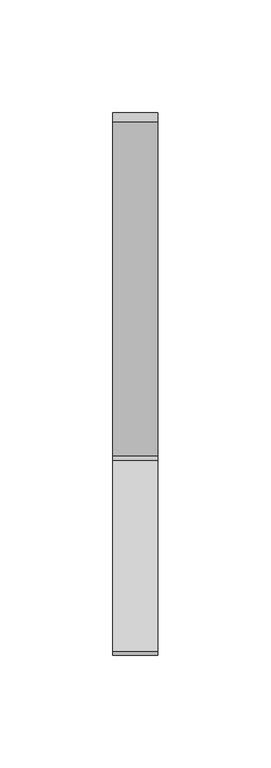
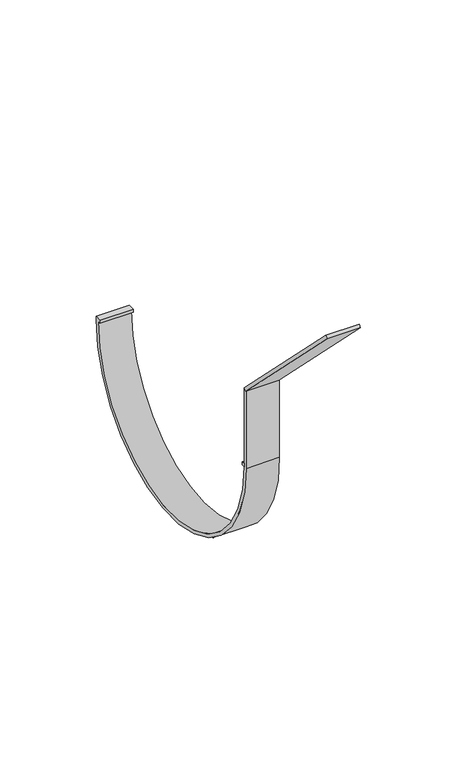
"""IFC4 building model written with IfcOpenShell, lengths in millimetres: proxy geometry, ➾ Кронштейн металлический : ➾ Кронштейн металлический."""

from ifc_helpers import new_model, si_unit, point, frame, origin, origin_with_axes, origin_2d, place, context, project, spatial, polyline, circle_curve, trimmed, segment, composite_curve, outline, extrude, source, transform, mapped, element, save


def generic_models_13adb273(model_context):
    return source(origin(), model_context, "Body", "SweptSolid", [
        extrude(outline(polyline([(0.0, -120.0), (0.0, 0.0), (20.0, 0.0), (20.0, -120.0), (0.0, -120.0)])), frame((10.0, -162.3670273, 133.4386002), z_axis=(0.0, 0.7071067811865492, 0.7071067811865459), x_axis=(-1.0, 0.0, 0.0)), (0.0, 0.0, 1.0), 2.0),
        extrude(outline(polyline([(-10.0, -74.1), (10.0, -74.1), (10.0, -76.1), (-10.0, -76.1), (-10.0, -74.1)])), origin_with_axes(), (0.0, 0.0, 1.0), 2.0),
        extrude(outline(composite_curve([segment(trimmed(circle_curve(origin_2d(), 76.1), [point((-76.1, 0.0))], [point((76.1, 0.0))], True, "CARTESIAN"), True, "CONTINUOUS"), segment(polyline([(76.1, 0.0), (74.055208, 0.0), (74.055208, 2.0), (78.1, 2.0), (78.1, 0.0)]), True, "CONTINUOUS"), segment(trimmed(circle_curve(origin_2d(), 78.1), [point((78.1, 0.0))], [point((-78.1, 0.0))], False, "CARTESIAN"), True, "CONTINUOUS"), segment(polyline([(-78.1, 0.0), (-78.1, 50.0), (-76.1, 50.0), (-76.1, 0.0)]), True, "CONTINUOUS")], self_intersect=False)), frame((-10.0, 0.0, 0.0), z_axis=(1.0, 0.0, 0.0), x_axis=(0.0, 1.0, 0.0)), (0.0, 0.0, 1.0), 20.0),
    ])


if __name__ == "__main__":
    model = new_model("IFC4")
    model_context = context("Model", 3, world=origin())
    ifc_project = project(units=[si_unit("LENGTHUNIT", "METRE", prefix="MILLI")], contexts=[model_context])
    site = spatial("IfcSite", under=ifc_project)
    building = spatial("IfcBuilding", under=site)
    placement = place(None, origin())
    generic_models_shape = generic_models_13adb273(model_context)
    element("IfcBuildingElementProxy", 1, Name="➾ Кронштейн металлический : ➾ Кронштейн металлический", ObjectType="➾ Кронштейн металлический : ➾ Кронштейн металлический", at=placement, inside=building, context=model_context, shape_type="MappedRepresentation", body=[
        mapped(generic_models_shape, transform((0.0, 0.0, 0.0), x_axis=(1.0, 0.0, 0.0), y_axis=(0.0, 1.0, 0.0), z_axis=(0.0, 0.0, 1.0))),
    ])
    save(model, "model.ifc")

# Revit data of these elements
# Type "➾ Кронштейн металлический : ➾ Кронштейн металлический"
#   Description = "Используется для монтажа желоба на\r\nкарнизе кровли. Крепится к стропильной\r\nсистеме или на скат кровли до монтажа\r\nкровельного покрытия"
#   Manufacturer = "ТехноНИКОЛЬ"
#   Model = "Комплектующие к водосточным системам"
#   URL = "https://tn-vodostok.ru/catalog/pvh/"
#   ADSK_Обозначение = "ТехноНИКОЛЬ"
#   ADSK_Наименование краткое = "Кронштейн"
#   ADSK_Наименование = "Кронштейн металлический"
#   ADSK_Масса_Текст = ""
#   ADSK_Марка = ""
#   ADSK_Код изделия = ""
#   ADSK_Завод-изготовитель = "ТехноНИКОЛЬ"
#   ADSK_Единица измерения = "шт."
#   ADSK_Группирование = "Комплектующие к водосточным системам"
#   ADSK_URL страницы изделия = "https://tn-vodostok.ru/catalog/pvh/"
#   ADSK_URL документации изделия = "https://tn-vodostok.ru/upload/iblock/c42/c427963cb77eb5c3c51f0cfb870e9e52.pdf"
#   Угол поворота кронштейна [instance default] = 45.00°
#   Длина пластины [instance default] = 250 mm
#   ADSK_Размер_Ширина = 20 mm
#   ADSK_Размер_Высота = 330 mm
#   ADSK_Количество = 1
#   Видимость [instance default] = yes
#   ADSK_Материал [instance default] = TN_Пластик_Коричневый_RAL8019
#   Default Elevation = 0
# Element 1 (IfcBuildingElementProxy, "➾ Кронштейн металлический : ➾ Кронштейн металлический")
#   Длина пластины = 50 mm
#   Materials on its faces: "TN_Пластик_Коричневый_RAL8019"
# Materials
#   "TN_Пластик_Коричневый_RAL8019": class "Типовые", colour RGB 61 54 53, transparency 0, Cost = 0
